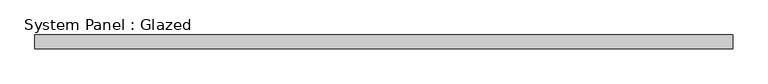
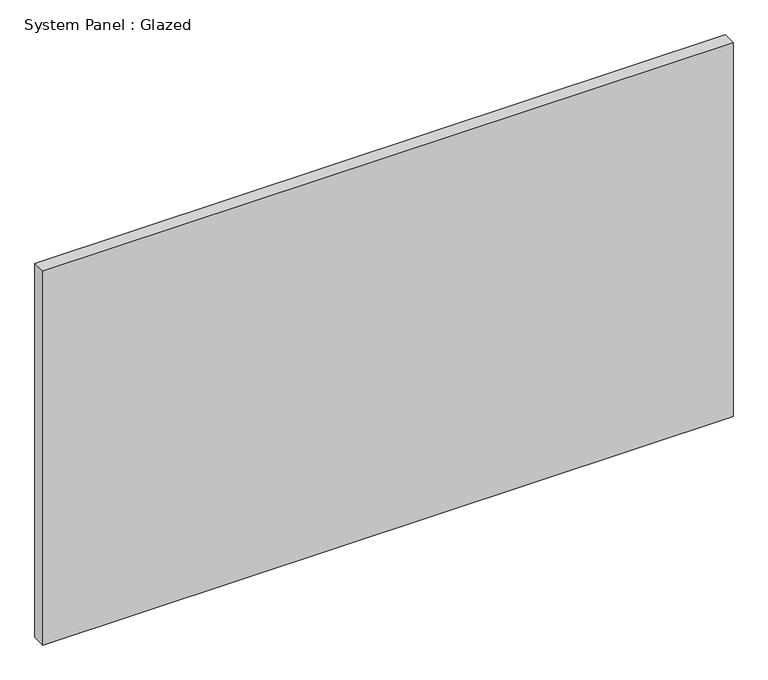
"""IFC4 building model written with IfcOpenShell, lengths in millimetres: plate geometry, System Panel : Glazed."""

from ifc_helpers import new_model, si_unit, origin, origin_with_axes, place, context, project, spatial, polyline, outline, extrude, source, transform, mapped, element, save


def system_panel_glazed_8e5047c4(model_context):
    return source(origin(), model_context, "Body", "SweptSolid", [
        extrude(outline(polyline([(632.4999999, 24.5), (-632.4999999, 24.5), (-632.4999999, 49.5), (632.4999999, 49.5), (632.4999999, 24.5)])), origin_with_axes(), (0.0, 0.0, 1.0), 725.0),
    ])


if __name__ == "__main__":
    model = new_model("IFC4")
    model_context = context("Model", 3, world=origin())
    ifc_project = project(units=[si_unit("LENGTHUNIT", "METRE", prefix="MILLI")], contexts=[model_context])
    site = spatial("IfcSite", under=ifc_project)
    building = spatial("IfcBuilding", under=site)
    placement = place(None, origin())
    system_panel_glazed_shape = system_panel_glazed_8e5047c4(model_context)
    element("IfcPlate", 1, ObjectType="System Panel : Glazed", at=placement, inside=building, context=model_context, shape_type="MappedRepresentation", body=[
        mapped(system_panel_glazed_shape, transform((0.0, 0.0, 0.0), x_axis=(1.0, 0.0, 0.0), y_axis=(0.0, 1.0, 0.0), z_axis=(0.0, 0.0, 1.0))),
    ])
    save(model, "model.ifc")

# Revit data of these elements
# Type "System Panel : Glazed"
#   Construction Type Id = "GSP4R"
#   Analytic Construction = "1/8 in Pilkington single glazing"
#   Visual Light Transmittance = 0.9
#   Solar Heat Gain Coefficient = 0.86
#   Heat Transfer Coefficient (U) = 6.7069 W/(m²·K)
#   Define Thermal Properties by = 1
# Element 1 (IfcPlate, "System Panel : Glazed")
#   Materials on its faces: "Glass"
# Materials
#   "Glass": class "Glass", colour RGB 0 128 192, transparency 0.9, Description = "Soda Lime Glass", Cost = 0
